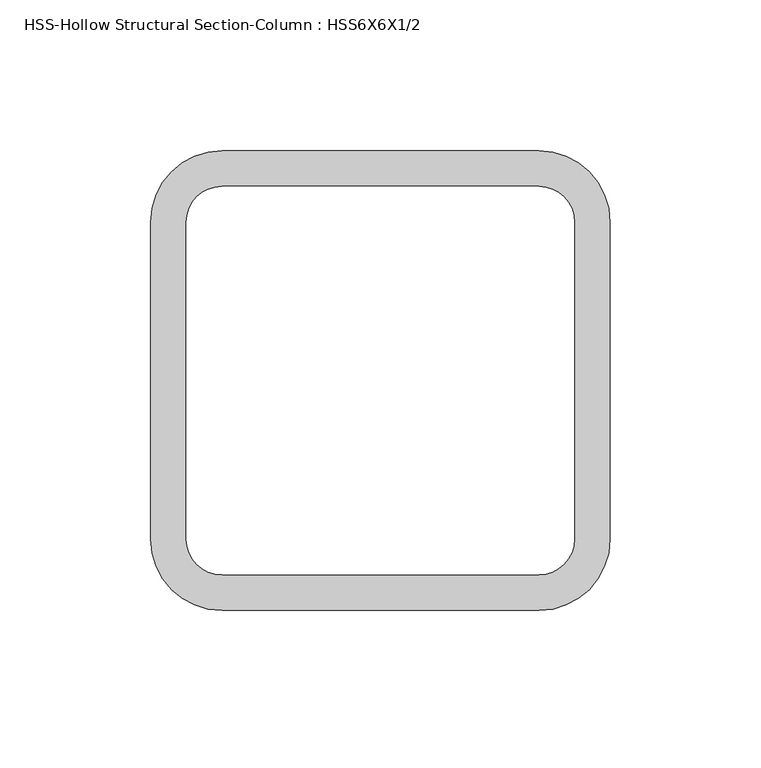
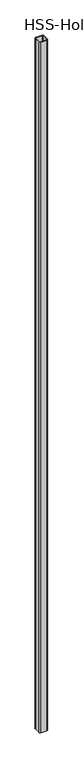
"""IFC4 building model written with IfcOpenShell, lengths in millimetres: column geometry, HSS-Hollow Structural Section-Column : HSS6X6X1/2."""

from ifc_helpers import new_model, si_unit, point, frame, frame_2d, origin, place, context, project, spatial, polyline, circle_curve, trimmed, segment, composite_curve, outline, extrude, source, transform, mapped, element, save


def hss_hollow_structural_section_column_hss6x6x1_2_08fbef70(model_context):
    return source(origin(), model_context, "Body", "SweptSolid", [
        extrude(outline(composite_curve([segment(trimmed(circle_curve(frame_2d((52.578, 52.578)), 23.622), [point((52.578, 76.2))], [point((76.2, 52.578))], False, "CARTESIAN"), True, "CONTINUOUS"), segment(polyline([(76.2, 52.578), (76.2, -52.578)]), True, "CONTINUOUS"), segment(trimmed(circle_curve(frame_2d((52.578, -52.578)), 23.622), [point((76.2, -52.578))], [point((52.578, -76.2))], False, "CARTESIAN"), True, "CONTINUOUS"), segment(polyline([(52.578, -76.2), (-52.578, -76.2)]), True, "CONTINUOUS"), segment(trimmed(circle_curve(frame_2d((-52.578, -52.578)), 23.622), [point((-52.578, -76.2))], [point((-76.2, -52.578))], False, "CARTESIAN"), True, "CONTINUOUS"), segment(polyline([(-76.2, -52.578), (-76.2, 52.578)]), True, "CONTINUOUS"), segment(trimmed(circle_curve(frame_2d((-52.578, 52.578)), 23.622), [point((-76.2, 52.578))], [point((-52.578, 76.2))], False, "CARTESIAN"), True, "CONTINUOUS"), segment(polyline([(-52.578, 76.2), (52.578, 76.2)]), True, "CONTINUOUS")], self_intersect=False), holes=[composite_curve([segment(polyline([(52.578, 64.389), (-52.578, 64.389)]), True, "CONTINUOUS"), segment(trimmed(circle_curve(frame_2d((-52.578, 52.578)), 11.811), [point((-52.578, 64.389))], [point((-64.389, 52.578))], True, "CARTESIAN"), True, "CONTINUOUS"), segment(polyline([(-64.389, 52.578), (-64.389, -52.578)]), True, "CONTINUOUS"), segment(trimmed(circle_curve(frame_2d((-52.578, -52.578)), 11.811), [point((-64.389, -52.578))], [point((-52.578, -64.389))], True, "CARTESIAN"), True, "CONTINUOUS"), segment(polyline([(-52.578, -64.389), (52.578, -64.389)]), True, "CONTINUOUS"), segment(trimmed(circle_curve(frame_2d((52.578, -52.578)), 11.811), [point((52.578, -64.389))], [point((64.389, -52.578))], True, "CARTESIAN"), True, "CONTINUOUS"), segment(polyline([(64.389, -52.578), (64.389, 52.578)]), True, "CONTINUOUS"), segment(trimmed(circle_curve(frame_2d((52.578, 52.578)), 11.811), [point((64.389, 52.578))], [point((52.578, 64.389))], True, "CARTESIAN"), True, "CONTINUOUS")], self_intersect=False)]), frame((0.0, 0.0, -609.6), z_axis=(0.0, 0.0, 1.0), x_axis=(1.0, 0.0, 0.0)), (0.0, 0.0, 1.0), 12979.4),
    ])


if __name__ == "__main__":
    model = new_model("IFC4")
    model_context = context("Model", 3, world=origin())
    ifc_project = project(units=[si_unit("LENGTHUNIT", "METRE", prefix="MILLI")], contexts=[model_context])
    site = spatial("IfcSite", under=ifc_project)
    building = spatial("IfcBuilding", under=site)
    placement = place(None, origin())
    hss_hollow_structural_section_column_hss6x6x1_2_shape = hss_hollow_structural_section_column_hss6x6x1_2_08fbef70(model_context)
    element("IfcColumn", 1, ObjectType="HSS-Hollow Structural Section-Column : HSS6X6X1/2", at=placement, inside=building, context=model_context, shape_type="MappedRepresentation", body=[
        mapped(hss_hollow_structural_section_column_hss6x6x1_2_shape, transform((0.0, 0.0, 0.0), x_axis=(1.0, 0.0, 0.0), y_axis=(0.0, 1.0, 0.0), z_axis=(0.0, 0.0, 1.0))),
    ])
    save(model, "model.ifc")

# Revit data of these elements
# Type "HSS-Hollow Structural Section-Column : HSS6X6X1/2"
#   Assembly Code = "B10"
#   Shape = "Square"
#   W = 35.1
#   Ht = 0' - 6"
#   b = 0' - 6"
#   kr = 0' - 0.93"
#   t = 0' - 0.465"
#   A = 0.0676389 SF
#   Structural Material [instance default] = Steel ASTM A500, Grade B, Rectangular and Square
# Element 1 (IfcColumn, "HSS-Hollow Structural Section-Column : HSS6X6X1/2")
#   Materials on its faces: "Steel ASTM A500, Grade B, Rectangular and Square"
# Materials
#   "Steel ASTM A500, Grade B, Rectangular and Square": class "Metal", colour RGB 199 199 199, transparency 0, Description = "Carbon steel", Cost = 0
